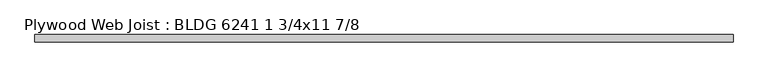
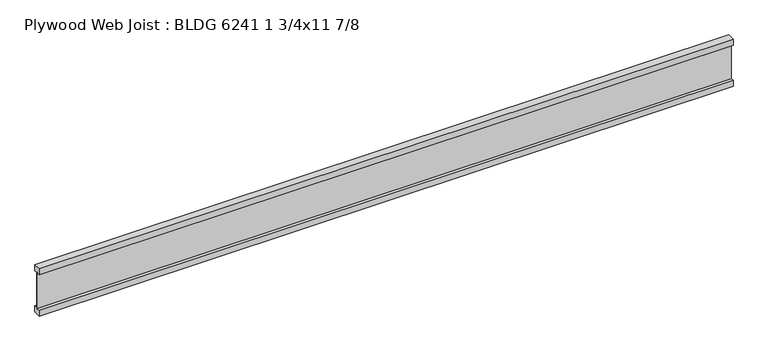
"""IFC4 building model written with IfcOpenShell, lengths in millimetres: beam geometry, Plywood Web Joist : BLDG 6241 1 3/4x11 7/8."""

import ifcopenshell
import ifcopenshell.guid

model = None  # the IFC model being written
_history = None  # IfcOwnerHistory: only IFC2X3 demands one
_inside = {}  # id of a spatial element -> (the spatial element, [elements in it])
_under = {}  # id of a project, library or spatial element -> (it, [spatial elements below it])
_declared = {}  # id of a project -> (the project, [libraries it declares])
_typed = {}  # id of a type object -> (the type object, [elements of that type])
_made_of = {}  # id of a material, layer set ... -> (it, [elements and type objects made of it])


def new_model(schema):
    """Start an empty IFC model of exactly this schema.

    Asked for "IFC4X3", IfcOpenShell would pick the latest addendum, in which some entities
    have other attributes; the version numbers below select the first issue.
    IFC2X3 requires an IfcOwnerHistory on every rooted entity: one is made here for all.
    """
    global model, _history
    if schema == "IFC4X3":
        model = ifcopenshell.file(schema_version=(4, 3, 0, 0))
    else:
        model = ifcopenshell.file(schema=schema)
    _inside.clear()
    _under.clear()
    _declared.clear()
    _typed.clear()
    _made_of.clear()
    _history = None
    if model.schema == "IFC2X3":
        org = make("IfcOrganization", Name="unknown")
        user = make(
            "IfcPersonAndOrganization",
            ThePerson=make("IfcPerson", FamilyName="unknown"),
            TheOrganization=org,
        )
        app = make(
            "IfcApplication",
            ApplicationDeveloper=org,
            Version="unknown",
            ApplicationFullName="unknown",
            ApplicationIdentifier="unknown",
        )
        _history = make(
            "IfcOwnerHistory",
            OwningUser=user,
            OwningApplication=app,
            ChangeAction="ADDED",
            CreationDate=0,
        )
    return model


def make(cls, **values):
    """One entity of the class cls with the attributes given. An attribute that is None is left unset."""
    return model.create_entity(
        cls, **{name: value for name, value in values.items() if value is not None}
    )


def rooted(cls, **values):
    """An entity with a GlobalId (a new one), such as an element, a storey or a relation."""
    return make(cls, GlobalId=ifcopenshell.guid.new(), OwnerHistory=_history, **values)


def si_unit(unit_type, name, prefix=None):
    """IfcSIUnit, for example si_unit("LENGTHUNIT", "METRE", prefix="MILLI")."""
    return make("IfcSIUnit", UnitType=unit_type, Prefix=prefix, Name=name)


def assignment(units):
    """IfcUnitAssignment: the units of a project."""
    return None if units is None else make("IfcUnitAssignment", Units=units)


def point(xyz):
    """IfcCartesianPoint."""
    return None if xyz is None else make("IfcCartesianPoint", Coordinates=xyz)


def direction(xyz):
    """IfcDirection."""
    return None if xyz is None else make("IfcDirection", DirectionRatios=xyz)


def frame(location, z_axis=None, x_axis=None):
    """IfcAxis2Placement3D, a coordinate frame: its origin and axes. An axis left out is left unset."""
    return make(
        "IfcAxis2Placement3D",
        Location=point(location),
        Axis=direction(z_axis),
        RefDirection=direction(x_axis),
    )


def origin():
    """The frame at (0, 0, 0) with its axes left unset."""
    return frame((0.0, 0.0, 0.0))


def place(relative_to, where):
    """IfcLocalPlacement: puts the frame where relative to a parent placement (None: the world)."""
    return make(
        "IfcLocalPlacement", PlacementRelTo=relative_to, RelativePlacement=where
    )


def context(
    kind, dimensions, precision=None, world=None, true_north=None, identifier=None
):
    """IfcGeometricRepresentationContext, for example the 3D "Model" context."""
    return make(
        "IfcGeometricRepresentationContext",
        ContextIdentifier=identifier,
        ContextType=kind,
        CoordinateSpaceDimension=dimensions,
        Precision=precision,
        WorldCoordinateSystem=world,
        TrueNorth=true_north,
    )


def project(units=None, contexts=None):
    """IfcProject with its units and contexts."""
    return rooted(
        "IfcProject",
        Name="project",
        RepresentationContexts=contexts,
        UnitsInContext=assignment(units),
    )


def spatial(cls, under=None, at=None, **own):
    """A site, building, storey or space (cls), placed at a placement, below another one or the project."""
    s = rooted(cls, ObjectPlacement=at, **own)
    if under is not None:
        _under.setdefault(under.id(), (under, []))[1].append(s)
    return s


def polyline(points):
    """IfcPolyline through the points."""
    return make("IfcPolyline", Points=[point(p) for p in points])


def outline(outer, holes=None, kind="AREA"):
    """IfcArbitraryClosedProfileDef: a profile drawn as a closed curve; with holes, ...WithVoids."""
    if holes is None:
        return make("IfcArbitraryClosedProfileDef", ProfileType=kind, OuterCurve=outer)
    return make(
        "IfcArbitraryProfileDefWithVoids",
        ProfileType=kind,
        OuterCurve=outer,
        InnerCurves=holes,
    )


def extrude(swept, where, along, depth):
    """IfcExtrudedAreaSolid: the profile swept, set in the frame where, extruded along a direction by depth."""
    return make(
        "IfcExtrudedAreaSolid",
        SweptArea=swept,
        Position=where,
        ExtrudedDirection=direction(along),
        Depth=depth,
    )


def shape(context_of_items, identifier, shape_type, items):
    """IfcShapeRepresentation: the items that make up one representation, for example the "Body"."""
    return make(
        "IfcShapeRepresentation",
        ContextOfItems=context_of_items,
        RepresentationIdentifier=identifier,
        RepresentationType=shape_type,
        Items=items,
    )


def source(mapping_origin, context_of_items, identifier, shape_type, items):
    """IfcRepresentationMap: a shape defined once, which mapped items show again and again."""
    return make(
        "IfcRepresentationMap",
        MappingOrigin=mapping_origin,
        MappedRepresentation=shape(context_of_items, identifier, shape_type, items),
    )


def transform(
    local_origin,
    x_axis=None,
    y_axis=None,
    z_axis=None,
    scale=None,
    scale2=None,
    scale3=None,
    uniform=True,
):
    """IfcCartesianTransformationOperator3D, or its non-uniform kind. x_axis, y_axis, z_axis: its Axis1, 2, 3."""
    if uniform:
        return make(
            "IfcCartesianTransformationOperator3D",
            Axis1=direction(x_axis),
            Axis2=direction(y_axis),
            LocalOrigin=point(local_origin),
            Scale=scale,
            Axis3=direction(z_axis),
        )
    return make(
        "IfcCartesianTransformationOperator3DnonUniform",
        Axis1=direction(x_axis),
        Axis2=direction(y_axis),
        LocalOrigin=point(local_origin),
        Scale=scale,
        Axis3=direction(z_axis),
        Scale2=scale2,
        Scale3=scale3,
    )


def mapped(mapping_source, mapping_target):
    """IfcMappedItem: shows the shape of a source again, moved by a transform."""
    return make(
        "IfcMappedItem", MappingSource=mapping_source, MappingTarget=mapping_target
    )


def made_of(thing, what):
    """Note that an element or type object is made of a material, layer set ...; save() writes the relation."""
    if what is not None:
        _made_of.setdefault(what.id(), (what, []))[1].append(thing)
    return thing


def element(
    cls,
    number,
    at=None,
    inside=None,
    cuts=None,
    type_object=None,
    material=None,
    context=None,
    identifier="Body",
    shape_type=None,
    held_by="IfcProductDefinitionShape",
    body=None,
    shapes=None,
    **own,
):
    """One element of the class cls, such as IfcWall. Its Tag is "e" and its number.

    at: its placement. inside: the storey or other place that contains it. cuts: it is an
    opening in that element (IfcRelVoidsElement). A single representation is given by context,
    identifier, shape_type and body (its items); several are given by shapes. held_by: the class
    of the entity that holds the representations. save() writes the other relations.
    """
    e = rooted(cls, Tag="e%d" % number, ObjectPlacement=at, **own)
    if body is not None:
        shapes = [shape(context, identifier, shape_type, body)]
    if shapes is not None:
        e.Representation = make(held_by, Representations=shapes)
    if inside is not None:
        _inside.setdefault(inside.id(), (inside, []))[1].append(e)
    if cuts is not None:
        rooted(
            "IfcRelVoidsElement", RelatingBuildingElement=cuts, RelatedOpeningElement=e
        )
    if type_object is not None:
        _typed.setdefault(type_object.id(), (type_object, []))[1].append(e)
    return made_of(e, material)


def aggregate(whole, parts):
    """IfcRelAggregates: a whole, such as a stair, and the parts it consists of."""
    return rooted("IfcRelAggregates", RelatingObject=whole, RelatedObjects=parts)


def save(model, path):
    """Write the relations noted so far, then the file.

    IfcRelAggregates (storeys below a building ...), IfcRelContainedInSpatialStructure (elements
    in a storey), IfcRelDefinesByType, IfcRelAssociatesMaterial and IfcRelDeclares: one each for
    every whole, place, type object, material and project.
    """
    for whole, parts in _under.values():
        aggregate(whole, parts)
    for where, things in _inside.values():
        rooted(
            "IfcRelContainedInSpatialStructure",
            RelatedElements=things,
            RelatingStructure=where,
        )
    for kind, things in _typed.values():
        rooted("IfcRelDefinesByType", RelatedObjects=things, RelatingType=kind)
    for what, things in _made_of.values():
        rooted("IfcRelAssociatesMaterial", RelatedObjects=things, RelatingMaterial=what)
    for by, libraries in _declared.values():
        rooted("IfcRelDeclares", RelatingContext=by, RelatedDefinitions=libraries)
    model.write(path)


def plywood_web_joist_bldg_6241_1_3_4x11_7_8_881987cb(model_context):
    return source(origin(), model_context, "Body", "SweptSolid", [
        extrude(outline(polyline([(-22.225, 150.8125), (22.225, 150.8125), (22.225, 112.7125), (4.7625, 112.7125), (4.7625, 119.0625), (-4.7625, 119.0625), (-4.7625, 112.7125), (-22.225, 112.7125), (-22.225, 150.8125)])), frame((-2121.2191036, 0.0, 0.0), z_axis=(1.0, 0.0, 0.0), x_axis=(0.0, 1.0, 0.0)), (0.0, 0.0, 1.0), 4201.8014143),
        extrude(outline(polyline([(22.225, -112.7125), (22.225, -150.8125), (-22.225, -150.8125), (-22.225, -112.7125), (-4.7625, -112.7125), (-4.7625, -118.3285374), (4.7625, -118.3285374), (4.7625, -112.7125), (22.225, -112.7125)])), frame((-2121.2191036, 0.0, 0.0), z_axis=(1.0, 0.0, 0.0), x_axis=(0.0, 1.0, 0.0)), (0.0, 0.0, 1.0), 4201.8014143),
        extrude(outline(polyline([(2080.5823107, 4.7625), (2080.5823107, -4.7625), (-2121.2191036, -4.7625), (-2121.2191036, 4.7625), (2080.5823107, 4.7625)])), frame((0.0, 0.0, -118.3285374), z_axis=(0.0, 0.0, 1.0), x_axis=(1.0, 0.0, 0.0)), (0.0, 0.0, 1.0), 237.3910374),
    ])


if __name__ == "__main__":
    model = new_model("IFC4")
    model_context = context("Model", 3, world=origin())
    ifc_project = project(units=[si_unit("LENGTHUNIT", "METRE", prefix="MILLI")], contexts=[model_context])
    site = spatial("IfcSite", under=ifc_project)
    building = spatial("IfcBuilding", under=site)
    placement = place(None, origin())
    plywood_web_joist_bldg_6241_1_3_4x11_7_8_shape = plywood_web_joist_bldg_6241_1_3_4x11_7_8_881987cb(model_context)
    element("IfcBeam", 1, ObjectType="Plywood Web Joist : BLDG 6241 1 3/4x11 7/8", at=placement, inside=building, context=model_context, shape_type="MappedRepresentation", body=[
        mapped(plywood_web_joist_bldg_6241_1_3_4x11_7_8_shape, transform((0.0, 0.0, 0.0), x_axis=(1.0, 0.0, 0.0), y_axis=(0.0, 1.0, 0.0), z_axis=(0.0, 0.0, 1.0))),
    ])
    save(model, "model.ifc")

# Revit data of these elements
# Type "Plywood Web Joist : BLDG 6241 1 3/4x11 7/8"
#   Assembly Code = "B10"
#   Length [instance default] = 5' - 0"
#   b = 0' - 1 3/4"
#   d = 0' - 11 7/8"
#   Structural Material [instance default] = Softwood, Lumber
# Element 1 (IfcBeam, "Plywood Web Joist : BLDG 6241 1 3/4x11 7/8")
#   Materials on its faces: "Softwood, Lumber"
# Materials
#   "Softwood, Lumber": class "Wood", colour RGB 223 192 134, transparency 0, Description = "Pinus Echinata", Cost = 0
